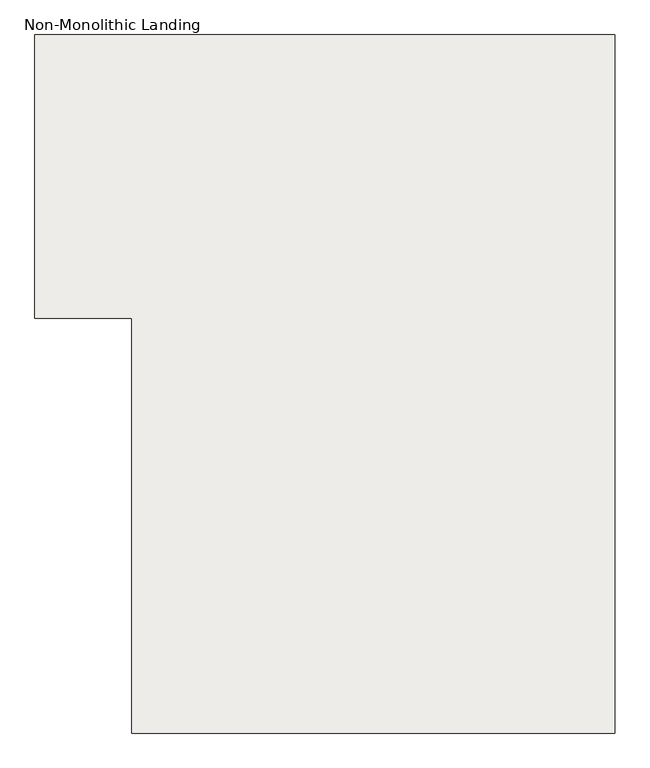
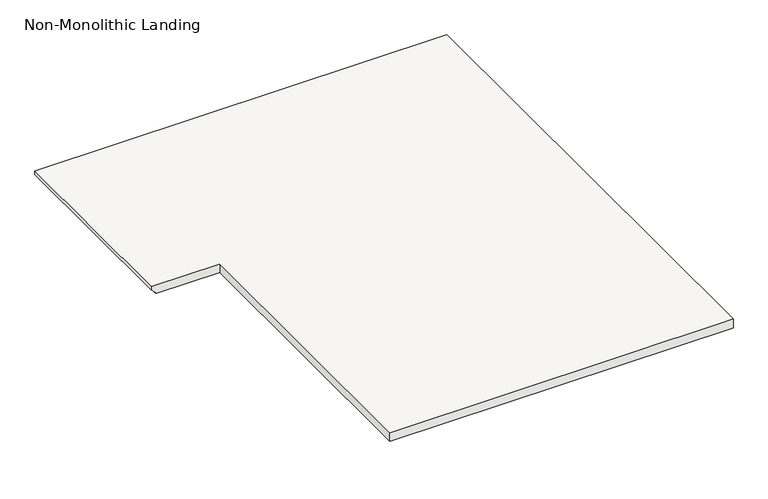
"""IFC4 building model written with IfcOpenShell, lengths in millimetres: slab geometry, Non-Monolithic Landing."""

from ifc_helpers import new_model, si_unit, origin, place, context, project, spatial, faceted_brep, source, transform, mapped, element, save


def non_monolithic_landing_a3dac32d(model_context):
    return source(origin(), model_context, "Body", "Brep", [
        faceted_brep([(-937.2122732, 8132.6265304, 0.0), (-937.2122732, 6497.5015304, 0.0), (967.7877268, 6497.5015304, 0.0), (967.7877268, 9250.2265304, 0.0), (-1318.2122732, 9250.2265304, 0.0), (-1318.2122732, 8132.6265304, 0.0), (-1292.8122732, 8132.6265304, -50.8), (-1292.8122732, 9250.2265304, -50.8), (967.7877268, 9250.2265304, -50.8), (967.7877268, 6497.5015304, -50.8), (-937.2122732, 6497.5015304, -50.8), (-937.2122732, 8132.6265304, -50.8), (-1292.8122732, 9250.2265304, -44.45), (-1318.2122732, 9250.2265304, -19.05), (-1318.2122732, 8132.6265304, -19.05), (-1292.8122732, 8132.6265304, -44.45)], [[[0, 1, 2, 3, 4, 5]], [[6, 7, 8, 9, 10, 11]], [[1, 0, 11, 10]], [[2, 1, 10, 9]], [[3, 2, 9, 8]], [[4, 3, 8, 7, 12, 13]], [[0, 5, 14, 15, 6, 11]], [[7, 6, 15, 12]], [[14, 5, 4, 13]], [[15, 14, 13, 12]]]),
    ])


if __name__ == "__main__":
    model = new_model("IFC4")
    model_context = context("Model", 3, world=origin())
    ifc_project = project(units=[si_unit("LENGTHUNIT", "METRE", prefix="MILLI")], contexts=[model_context])
    site = spatial("IfcSite", under=ifc_project)
    building = spatial("IfcBuilding", under=site)
    placement = place(None, origin())
    non_monolithic_landing_shape = non_monolithic_landing_a3dac32d(model_context)
    element("IfcSlab", 1, ObjectType="Non-Monolithic Landing", at=placement, inside=building, context=model_context, shape_type="MappedRepresentation", body=[
        mapped(non_monolithic_landing_shape, transform((0.0, 0.0, 0.0), x_axis=(1.0, 0.0, 0.0), y_axis=(0.0, 1.0, 0.0), z_axis=(0.0, 0.0, 1.0))),
    ])
    save(model, "model.ifc")
